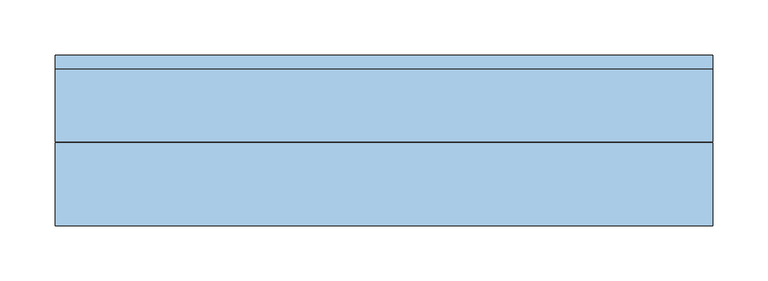
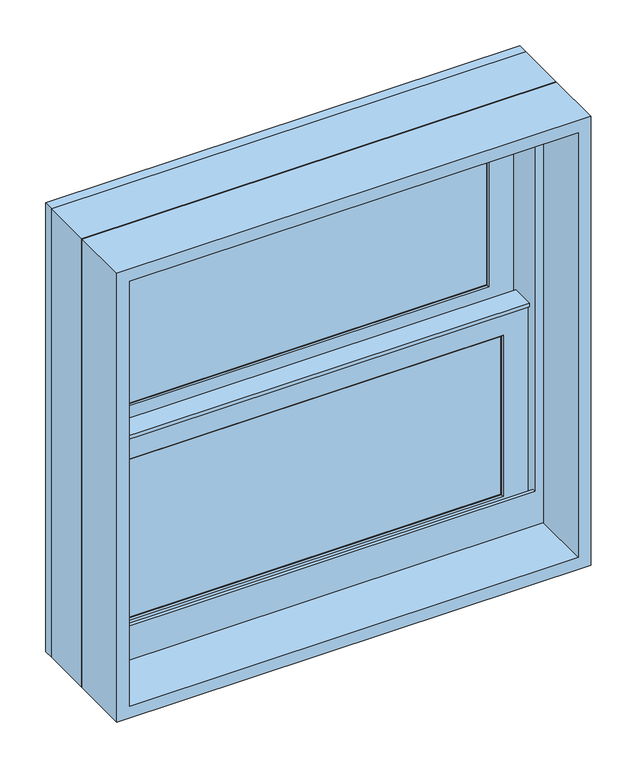
"""IFC4 building model written with IfcOpenShell, lengths in millimetres: window geometry, Window-Double_Hung-Marvin-Essential : ESDH2020."""

import ifcopenshell
import ifcopenshell.guid

model = None  # the IFC model being written
_history = None  # IfcOwnerHistory: only IFC2X3 demands one
_inside = {}  # id of a spatial element -> (the spatial element, [elements in it])
_under = {}  # id of a project, library or spatial element -> (it, [spatial elements below it])
_declared = {}  # id of a project -> (the project, [libraries it declares])
_typed = {}  # id of a type object -> (the type object, [elements of that type])
_made_of = {}  # id of a material, layer set ... -> (it, [elements and type objects made of it])


def new_model(schema):
    """Start an empty IFC model of exactly this schema.

    Asked for "IFC4X3", IfcOpenShell would pick the latest addendum, in which some entities
    have other attributes; the version numbers below select the first issue.
    IFC2X3 requires an IfcOwnerHistory on every rooted entity: one is made here for all.
    """
    global model, _history
    if schema == "IFC4X3":
        model = ifcopenshell.file(schema_version=(4, 3, 0, 0))
    else:
        model = ifcopenshell.file(schema=schema)
    _inside.clear()
    _under.clear()
    _declared.clear()
    _typed.clear()
    _made_of.clear()
    _history = None
    if model.schema == "IFC2X3":
        org = make("IfcOrganization", Name="unknown")
        user = make(
            "IfcPersonAndOrganization",
            ThePerson=make("IfcPerson", FamilyName="unknown"),
            TheOrganization=org,
        )
        app = make(
            "IfcApplication",
            ApplicationDeveloper=org,
            Version="unknown",
            ApplicationFullName="unknown",
            ApplicationIdentifier="unknown",
        )
        _history = make(
            "IfcOwnerHistory",
            OwningUser=user,
            OwningApplication=app,
            ChangeAction="ADDED",
            CreationDate=0,
        )
    return model


def make(cls, **values):
    """One entity of the class cls with the attributes given. An attribute that is None is left unset."""
    return model.create_entity(
        cls, **{name: value for name, value in values.items() if value is not None}
    )


def rooted(cls, **values):
    """An entity with a GlobalId (a new one), such as an element, a storey or a relation."""
    return make(cls, GlobalId=ifcopenshell.guid.new(), OwnerHistory=_history, **values)


def si_unit(unit_type, name, prefix=None):
    """IfcSIUnit, for example si_unit("LENGTHUNIT", "METRE", prefix="MILLI")."""
    return make("IfcSIUnit", UnitType=unit_type, Prefix=prefix, Name=name)


def assignment(units):
    """IfcUnitAssignment: the units of a project."""
    return None if units is None else make("IfcUnitAssignment", Units=units)


def point(xyz):
    """IfcCartesianPoint."""
    return None if xyz is None else make("IfcCartesianPoint", Coordinates=xyz)


def direction(xyz):
    """IfcDirection."""
    return None if xyz is None else make("IfcDirection", DirectionRatios=xyz)


def frame(location, z_axis=None, x_axis=None):
    """IfcAxis2Placement3D, a coordinate frame: its origin and axes. An axis left out is left unset."""
    return make(
        "IfcAxis2Placement3D",
        Location=point(location),
        Axis=direction(z_axis),
        RefDirection=direction(x_axis),
    )


def origin():
    """The frame at (0, 0, 0) with its axes left unset."""
    return frame((0.0, 0.0, 0.0))


def place(relative_to, where):
    """IfcLocalPlacement: puts the frame where relative to a parent placement (None: the world)."""
    return make(
        "IfcLocalPlacement", PlacementRelTo=relative_to, RelativePlacement=where
    )


def context(
    kind, dimensions, precision=None, world=None, true_north=None, identifier=None
):
    """IfcGeometricRepresentationContext, for example the 3D "Model" context."""
    return make(
        "IfcGeometricRepresentationContext",
        ContextIdentifier=identifier,
        ContextType=kind,
        CoordinateSpaceDimension=dimensions,
        Precision=precision,
        WorldCoordinateSystem=world,
        TrueNorth=true_north,
    )


def project(units=None, contexts=None):
    """IfcProject with its units and contexts."""
    return rooted(
        "IfcProject",
        Name="project",
        RepresentationContexts=contexts,
        UnitsInContext=assignment(units),
    )


def spatial(cls, under=None, at=None, **own):
    """A site, building, storey or space (cls), placed at a placement, below another one or the project."""
    s = rooted(cls, ObjectPlacement=at, **own)
    if under is not None:
        _under.setdefault(under.id(), (under, []))[1].append(s)
    return s


def polyline(points):
    """IfcPolyline through the points."""
    return make("IfcPolyline", Points=[point(p) for p in points])


def outline(outer, holes=None, kind="AREA"):
    """IfcArbitraryClosedProfileDef: a profile drawn as a closed curve; with holes, ...WithVoids."""
    if holes is None:
        return make("IfcArbitraryClosedProfileDef", ProfileType=kind, OuterCurve=outer)
    return make(
        "IfcArbitraryProfileDefWithVoids",
        ProfileType=kind,
        OuterCurve=outer,
        InnerCurves=holes,
    )


def extrude(swept, where, along, depth):
    """IfcExtrudedAreaSolid: the profile swept, set in the frame where, extruded along a direction by depth."""
    return make(
        "IfcExtrudedAreaSolid",
        SweptArea=swept,
        Position=where,
        ExtrudedDirection=direction(along),
        Depth=depth,
    )


def faces_of(points, faces, orient=None, outer=None):
    """IfcFace entities. A face is a list of loops; a loop is a list of indices into points, from 0.

    orient and outer hold one flag for each loop. By default every Orientation is true, the
    first loop of a face is its IfcFaceOuterBound and the others are IfcFaceBound.
    """
    made = []
    for i, loops in enumerate(faces):
        bounds = []
        for j, loop in enumerate(loops):
            is_outer = j == 0 if outer is None else outer[i][j]
            bounds.append(
                make(
                    "IfcFaceOuterBound" if is_outer else "IfcFaceBound",
                    Bound=make("IfcPolyLoop", Polygon=[points[k] for k in loop]),
                    Orientation=True if orient is None else orient[i][j],
                )
            )
        made.append(make("IfcFace", Bounds=bounds))
    return made


def faceted_brep(points, faces, orient=None, outer=None, voids=None):
    """IfcFacetedBrep: a solid bounded by flat faces; with voids (closed shells), ...WithVoids."""
    shared = [point(p) for p in points]
    hull = make("IfcClosedShell", CfsFaces=faces_of(shared, faces, orient, outer))
    if voids is None:
        return make("IfcFacetedBrep", Outer=hull)
    return make(
        "IfcFacetedBrepWithVoids",
        Outer=hull,
        Voids=[
            make(cls, CfsFaces=faces_of(shared, fs, o, b)) for cls, fs, o, b in voids
        ],
    )


def shape(context_of_items, identifier, shape_type, items):
    """IfcShapeRepresentation: the items that make up one representation, for example the "Body"."""
    return make(
        "IfcShapeRepresentation",
        ContextOfItems=context_of_items,
        RepresentationIdentifier=identifier,
        RepresentationType=shape_type,
        Items=items,
    )


def source(mapping_origin, context_of_items, identifier, shape_type, items):
    """IfcRepresentationMap: a shape defined once, which mapped items show again and again."""
    return make(
        "IfcRepresentationMap",
        MappingOrigin=mapping_origin,
        MappedRepresentation=shape(context_of_items, identifier, shape_type, items),
    )


def transform(
    local_origin,
    x_axis=None,
    y_axis=None,
    z_axis=None,
    scale=None,
    scale2=None,
    scale3=None,
    uniform=True,
):
    """IfcCartesianTransformationOperator3D, or its non-uniform kind. x_axis, y_axis, z_axis: its Axis1, 2, 3."""
    if uniform:
        return make(
            "IfcCartesianTransformationOperator3D",
            Axis1=direction(x_axis),
            Axis2=direction(y_axis),
            LocalOrigin=point(local_origin),
            Scale=scale,
            Axis3=direction(z_axis),
        )
    return make(
        "IfcCartesianTransformationOperator3DnonUniform",
        Axis1=direction(x_axis),
        Axis2=direction(y_axis),
        LocalOrigin=point(local_origin),
        Scale=scale,
        Axis3=direction(z_axis),
        Scale2=scale2,
        Scale3=scale3,
    )


def mapped(mapping_source, mapping_target):
    """IfcMappedItem: shows the shape of a source again, moved by a transform."""
    return make(
        "IfcMappedItem", MappingSource=mapping_source, MappingTarget=mapping_target
    )


def made_of(thing, what):
    """Note that an element or type object is made of a material, layer set ...; save() writes the relation."""
    if what is not None:
        _made_of.setdefault(what.id(), (what, []))[1].append(thing)
    return thing


def element(
    cls,
    number,
    at=None,
    inside=None,
    cuts=None,
    type_object=None,
    material=None,
    context=None,
    identifier="Body",
    shape_type=None,
    held_by="IfcProductDefinitionShape",
    body=None,
    shapes=None,
    **own,
):
    """One element of the class cls, such as IfcWall. Its Tag is "e" and its number.

    at: its placement. inside: the storey or other place that contains it. cuts: it is an
    opening in that element (IfcRelVoidsElement). A single representation is given by context,
    identifier, shape_type and body (its items); several are given by shapes. held_by: the class
    of the entity that holds the representations. save() writes the other relations.
    """
    e = rooted(cls, Tag="e%d" % number, ObjectPlacement=at, **own)
    if body is not None:
        shapes = [shape(context, identifier, shape_type, body)]
    if shapes is not None:
        e.Representation = make(held_by, Representations=shapes)
    if inside is not None:
        _inside.setdefault(inside.id(), (inside, []))[1].append(e)
    if cuts is not None:
        rooted(
            "IfcRelVoidsElement", RelatingBuildingElement=cuts, RelatedOpeningElement=e
        )
    if type_object is not None:
        _typed.setdefault(type_object.id(), (type_object, []))[1].append(e)
    return made_of(e, material)


def aggregate(whole, parts):
    """IfcRelAggregates: a whole, such as a stair, and the parts it consists of."""
    return rooted("IfcRelAggregates", RelatingObject=whole, RelatedObjects=parts)


def save(model, path):
    """Write the relations noted so far, then the file.

    IfcRelAggregates (storeys below a building ...), IfcRelContainedInSpatialStructure (elements
    in a storey), IfcRelDefinesByType, IfcRelAssociatesMaterial and IfcRelDeclares: one each for
    every whole, place, type object, material and project.
    """
    for whole, parts in _under.values():
        aggregate(whole, parts)
    for where, things in _inside.values():
        rooted(
            "IfcRelContainedInSpatialStructure",
            RelatedElements=things,
            RelatingStructure=where,
        )
    for kind, things in _typed.values():
        rooted("IfcRelDefinesByType", RelatedObjects=things, RelatingType=kind)
    for what, things in _made_of.values():
        rooted("IfcRelAssociatesMaterial", RelatedObjects=things, RelatingMaterial=what)
    for by, libraries in _declared.values():
        rooted("IfcRelDeclares", RelatingContext=by, RelatedDefinitions=libraries)
    model.write(path)


def window_35121546(model_context):
    return source(origin(), model_context, "Body", "SolidModel", [
        extrude(outline(polyline([(89.9583333, 20.6375), (89.9583333, 15.875), (70.9083333, 15.875), (70.9083333, 20.6375), (89.9583333, 20.6375)])), frame((0.0, 0.0, 1898.65), z_axis=(0.0, 0.0, 1.0), x_axis=(1.0, 0.0, 0.0)), (0.0, 0.0, 1.0), 222.25),
        extrude(outline(polyline([(-70.9083333, 20.6375), (-70.9083333, 15.875), (-89.9583333, 15.875), (-89.9583333, 20.6375), (-70.9083333, 20.6375)])), frame((0.0, 0.0, 1898.65), z_axis=(0.0, 0.0, 1.0), x_axis=(1.0, 0.0, 0.0)), (0.0, 0.0, 1.0), 222.25),
        extrude(outline(polyline([(241.3, 20.6375), (241.3, 15.875), (-241.3, 15.875), (-241.3, 20.6375), (241.3, 20.6375)])), frame((0.0, 0.0, 2000.25), z_axis=(0.0, 0.0, 1.0), x_axis=(1.0, 0.0, 0.0)), (0.0, 0.0, 1.0), 19.05),
        extrude(outline(polyline([(-89.9583333, 46.83125), (-89.9583333, 51.59375), (-70.9083333, 51.59375), (-70.9083333, 46.83125), (-89.9583333, 46.83125)])), frame((0.0, 0.0, 2159.0), z_axis=(0.0, 0.0, 1.0), x_axis=(1.0, 0.0, 0.0)), (0.0, 0.0, 1.0), 222.25),
        extrude(outline(polyline([(70.9083333, 46.83125), (70.9083333, 51.59375), (89.9583333, 51.59375), (89.9583333, 46.83125), (70.9083333, 46.83125)])), frame((0.0, 0.0, 2159.0), z_axis=(0.0, 0.0, 1.0), x_axis=(1.0, 0.0, 0.0)), (0.0, 0.0, 1.0), 222.25),
        extrude(outline(polyline([(-241.3, 46.83125), (-241.3, 51.59375), (241.3, 51.59375), (241.3, 46.83125), (-241.3, 46.83125)])), frame((0.0, 0.0, 2260.6), z_axis=(0.0, 0.0, 1.0), x_axis=(1.0, 0.0, 0.0)), (0.0, 0.0, 1.0), 19.05),
        extrude(outline(polyline([(89.9583333, 20.6375), (70.9083333, 20.6375), (70.9083333, 25.4), (89.9583333, 25.4), (89.9583333, 20.6375)])), frame((0.0, 0.0, 1898.65), z_axis=(0.0, 0.0, 1.0), x_axis=(1.0, 0.0, 0.0)), (0.0, 0.0, 1.0), 222.25),
        extrude(outline(polyline([(-70.9083333, 20.6375), (-89.9583333, 20.6375), (-89.9583333, 25.4), (-70.9083333, 25.4), (-70.9083333, 20.6375)])), frame((0.0, 0.0, 1898.65), z_axis=(0.0, 0.0, 1.0), x_axis=(1.0, 0.0, 0.0)), (0.0, 0.0, 1.0), 222.25),
        extrude(outline(polyline([(241.3, 20.6375), (-241.3, 20.6375), (-241.3, 25.4), (241.3, 25.4), (241.3, 20.6375)])), frame((0.0, 0.0, 2000.25), z_axis=(0.0, 0.0, 1.0), x_axis=(1.0, 0.0, 0.0)), (0.0, 0.0, 1.0), 19.05),
        extrude(outline(polyline([(-89.9583333, 56.35625), (-70.9083333, 56.35625), (-70.9083333, 51.59375), (-89.9583333, 51.59375), (-89.9583333, 56.35625)])), frame((0.0, 0.0, 2159.0), z_axis=(0.0, 0.0, 1.0), x_axis=(1.0, 0.0, 0.0)), (0.0, 0.0, 1.0), 222.25),
        extrude(outline(polyline([(70.9083333, 56.35625), (89.9583333, 56.35625), (89.9583333, 51.59375), (70.9083333, 51.59375), (70.9083333, 56.35625)])), frame((0.0, 0.0, 2159.0), z_axis=(0.0, 0.0, 1.0), x_axis=(1.0, 0.0, 0.0)), (0.0, 0.0, 1.0), 222.25),
        extrude(outline(polyline([(-241.3, 56.35625), (241.3, 56.35625), (241.3, 51.59375), (-241.3, 51.59375), (-241.3, 56.35625)])), frame((0.0, 0.0, 2260.6), z_axis=(0.0, 0.0, 1.0), x_axis=(1.0, 0.0, 0.0)), (0.0, 0.0, 1.0), 19.05),
        faceted_brep([(-268.2875, 5.6780605, 2150.9351748), (-268.2875, 5.6780605, 2146.3), (268.2875, 5.6780605, 2146.3), (268.2875, 5.6780605, 2150.9351748), (-268.2875, 34.8118605, 2150.9351748), (268.2875, 34.8118605, 2150.9351748), (268.2875, 34.8118605, 2146.3), (-268.2875, 34.8118605, 2146.3), (-268.2875, 30.1625, 2146.3), (-268.2875, 30.1625, 1871.6625), (-268.2875, 8.9241104, 1871.6625), (-268.2875, 8.9241104, 2146.3), (268.2875, 8.9241104, 2146.3), (268.2875, 30.1625, 2146.3), (268.2875, 8.9241104, 1871.6625), (268.2875, 30.1625, 1871.6625), (-252.4034752, 11.90625, 2132.0034752), (-252.4034752, 30.1625, 2132.0034752), (252.4034752, 30.1625, 2132.0034752), (252.4034752, 11.90625, 2132.0034752), (-235.74375, 10.4662439, 2115.34375), (-235.74375, 11.90625, 2115.34375), (235.74375, 11.90625, 2115.34375), (235.74375, 10.4662439, 2115.34375), (237.2858834, 8.9241104, 2116.8858834), (-237.2858834, 8.9241104, 2116.8858834), (252.4034752, 30.1625, 1887.5465248), (252.4034752, 11.90625, 1887.5465248), (235.74375, 11.90625, 1904.20625), (235.74375, 10.4662439, 1904.20625), (237.2858834, 8.9241104, 1902.6641166), (-252.4034752, 30.1625, 1887.5465248), (-252.4034752, 11.90625, 1887.5465248), (-235.74375, 11.90625, 1904.20625), (-235.74375, 10.4662439, 1904.20625), (-237.2858834, 8.9241104, 1902.6641166)], [[[0, 1, 2, 3]], [[4, 5, 6, 7]], [[1, 0, 4, 7, 8, 9, 10, 11]], [[2, 1, 11, 12]], [[7, 6, 13, 8]], [[3, 2, 12, 14, 15, 13, 6, 5]], [[0, 3, 5, 4]], [[16, 17, 18, 19]], [[20, 21, 22, 23]], [[20, 23, 24, 25]], [[19, 18, 26, 27]], [[23, 22, 28, 29]], [[24, 23, 29, 30]], [[27, 26, 31, 32]], [[29, 28, 33, 34]], [[30, 29, 34, 35]], [[15, 14, 10, 9]], [[15, 9, 8, 13], [18, 17, 31, 26]], [[17, 16, 32, 31]], [[16, 19, 27, 32], [22, 21, 33, 28]], [[21, 20, 34, 33]], [[20, 25, 35, 34]], [[10, 14, 12, 11], [25, 24, 30, 35]]]),
        extrude(outline(polyline([(38.5955581, 2132.0125), (33.5778968, 2132.0125), (33.5778968, 2133.6), (39.9405976, 2133.6), (39.9405976, 2132.0125), (61.515625, 2132.0125), (47.6307501, 2128.6975159), (38.5955581, 2128.6975159), (38.5955581, 2132.0125)])), frame((-268.2875, 0.0, 0.0), z_axis=(1.0, 0.0, 0.0), x_axis=(0.0, 1.0, 0.0)), (0.0, 0.0, 1.0), 536.575),
        faceted_brep([(298.45, 0.0, 1841.5), (298.45, 0.0, 2438.4), (-298.45, 0.0, 2438.4), (-298.45, 0.0, 1841.5), (272.25625, 0.0, 1902.61875), (-272.25625, 0.0, 1902.61875), (-272.25625, 0.0, 2412.20625), (272.25625, 0.0, 2412.20625), (272.25625, 3.96875, 1841.5), (-272.25625, 3.96875, 1841.5), (-272.25625, 3.96875, 1902.61875), (272.25625, 3.96875, 1902.61875), (-298.45, 65.6828125, 1841.5), (-272.25625, 65.6828125, 1841.5), (272.25625, 65.6828125, 1841.5), (298.45, 65.6828125, 1841.5), (-298.45, 65.6828125, 2438.4), (298.45, 65.6828125, 2438.4), (272.25625, 65.6828125, 2412.20625), (-272.25625, 65.6828125, 2412.20625)], [[[0, 1, 2, 3], [4, 5, 6, 7]], [[8, 9, 10, 11]], [[5, 4, 11, 10]], [[0, 3, 12, 13, 9, 8, 14, 15]], [[13, 12, 16, 17, 15, 14, 18, 19]], [[13, 19, 6, 5, 10, 9]], [[7, 6, 19, 18]], [[18, 14, 8, 11, 4, 7]], [[1, 0, 15, 17]], [[2, 1, 17, 16]], [[3, 2, 16, 12]]]),
        faceted_brep([(272.25625, 30.1625, 2139.95), (270.66875, 30.1625, 2139.95), (270.66875, 30.1625, 1865.8544613), (272.25625, 30.1625, 1865.8544613), (-270.66875, 30.1625, 2139.95), (-272.25625, 30.1625, 2139.95), (-272.25625, 30.1625, 1865.8544613), (-270.66875, 30.1625, 1865.8544613), (270.66875, 63.5, 2139.95), (272.25625, 63.5, 2139.95), (272.25625, 63.5, 1859.3743077), (270.66875, 63.5, 1859.3743077), (-272.25625, 63.5, 2139.95), (-270.66875, 63.5, 2139.95), (-270.66875, 63.5, 1859.3743077), (-272.25625, 63.5, 1859.3743077), (283.5108932, 3.96875, 1870.9460105), (283.5108932, 3.96875, 1841.5), (283.5108932, 65.6828125, 1841.5), (283.5108932, 65.6828125, 1858.950012), (-283.5108932, 3.96875, 1841.5), (-283.5108932, 3.96875, 1870.9460105), (-283.5108932, 65.6828125, 1858.950012), (-283.5108932, 65.6828125, 1841.5), (283.5108932, 78.58125, 1856.4428097), (-283.5108932, 78.58125, 1856.4428097), (-281.4971252, 68.2348864, 1858.4539391), (-263.53135, 68.2348864, 1858.4539391), (-263.53135, 65.6828125, 1858.950012), (263.53135, 65.6828125, 1858.950012), (263.53135, 68.2348864, 1858.4539391), (281.4971252, 68.2348864, 1858.4539391), (-298.45, 65.6828125, 1841.5), (-298.45, 78.5948249, 1841.5), (298.45, 78.5948249, 1841.5), (298.45, 65.6828125, 1841.5), (-298.45, 78.58125, 2438.4), (298.45, 78.58125, 2438.4), (283.5108932, 78.58125, 2423.4608932), (-283.5108932, 78.58125, 2423.4608932), (-298.45, 65.6828125, 2438.4), (-281.4971252, 68.2348864, 2421.4471252), (281.4971252, 68.2348864, 2421.4471252), (263.53135, 68.2348864, 2403.48135), (-263.53135, 68.2348864, 2403.48135), (-263.53135, 65.6828125, 2403.48135), (263.53135, 65.6828125, 2403.48135), (298.45, 65.6828125, 2438.4)], [[[0, 1, 2, 3]], [[4, 5, 6, 7]], [[8, 9, 10, 11]], [[12, 13, 14, 15]], [[1, 8, 11, 2]], [[9, 0, 3, 10]], [[1, 0, 9, 8]], [[5, 4, 13, 12]], [[5, 12, 15, 6]], [[13, 4, 7, 14]], [[16, 17, 18, 19]], [[20, 21, 22, 23]], [[24, 25, 26, 27, 28, 22, 21, 16, 19, 29, 30, 31], [3, 2, 11, 10], [7, 6, 15, 14]], [[17, 16, 21, 20]], [[17, 20, 23, 32, 33, 34, 35, 18]], [[34, 33, 36, 37], [25, 24, 38, 39]], [[33, 32, 40, 36]], [[39, 41, 26, 25]], [[41, 42, 31, 30, 43, 44, 27, 26]], [[44, 45, 28, 27]], [[40, 32, 23, 22, 28, 45, 46, 29, 19, 18, 35, 47]], [[36, 40, 47, 37]], [[39, 38, 42, 41]], [[44, 43, 46, 45]], [[34, 37, 47, 35]], [[42, 38, 24, 31]], [[46, 43, 30, 29]]]),
        extrude(outline(polyline([(248.44375, 11.90625), (-248.44375, 11.90625), (-248.44375, 15.08125), (248.44375, 15.08125), (248.44375, 11.90625)])), frame((0.0, 0.0, 1891.50625), z_axis=(0.0, 0.0, 1.0), x_axis=(1.0, 0.0, 0.0)), (0.0, 0.0, 1.0), 236.5375),
        extrude(outline(polyline([(248.44375, 42.8625), (-248.44375, 42.8625), (-248.44375, 46.0375), (248.44375, 46.0375), (248.44375, 42.8625)])), frame((0.0, 0.0, 2151.85625), z_axis=(0.0, 0.0, 1.0), x_axis=(1.0, 0.0, 0.0)), (0.0, 0.0, 1.0), 236.5375),
        faceted_brep([(-235.74375, 31.194477, 2115.34375), (-237.2858834, 32.7366104, 2116.8858834), (237.2858834, 32.7366104, 2116.8858834), (235.74375, 31.194477, 2115.34375), (-235.74375, 30.1625, 2115.34375), (235.74375, 30.1625, 2115.34375), (-268.2875, 32.7366104, 2147.8875), (-268.2875, 30.1625, 2147.8875), (268.2875, 30.1625, 2147.8875), (268.2875, 32.7366104, 2147.8875), (237.2858834, 32.7366104, 1902.6641166), (235.74375, 31.194477, 1904.20625), (235.74375, 30.1625, 1904.20625), (268.2875, 30.1625, 1871.6625), (268.2875, 32.7366104, 1871.6625), (-237.2858834, 32.7366104, 1902.6641166), (-235.74375, 31.194477, 1904.20625), (-235.74375, 30.1625, 1904.20625), (-268.2875, 30.1625, 1871.6625), (-268.2875, 32.7366104, 1871.6625)], [[[0, 1, 2, 3]], [[4, 0, 3, 5]], [[6, 7, 8, 9]], [[3, 2, 10, 11]], [[5, 3, 11, 12]], [[9, 8, 13, 14]], [[11, 10, 15, 16]], [[12, 11, 16, 17]], [[14, 13, 18, 19]], [[9, 14, 19, 6], [1, 15, 10, 2]], [[16, 15, 1, 0]], [[17, 16, 0, 4]], [[7, 18, 13, 8], [5, 12, 17, 4]], [[19, 18, 7, 6]]]),
        faceted_brep([(-252.4034752, 42.8625, 2392.3534752), (-252.4034752, 61.11875, 2392.3534752), (252.4034752, 61.11875, 2392.3534752), (252.4034752, 42.8625, 2392.3534752), (-235.74375, 41.4224939, 2375.69375), (-235.74375, 42.8625, 2375.69375), (235.74375, 42.8625, 2375.69375), (235.74375, 41.4224939, 2375.69375), (-237.2858834, 39.8803604, 2377.2358834), (237.2858834, 39.8803604, 2377.2358834), (-268.2875, 61.11875, 2408.2375), (-268.2875, 39.8803604, 2408.2375), (268.2875, 39.8803604, 2408.2375), (268.2875, 61.11875, 2408.2375), (252.4034752, 61.11875, 2147.8965248), (252.4034752, 42.8625, 2147.8965248), (235.74375, 42.8625, 2164.55625), (235.74375, 41.4224939, 2164.55625), (237.2858834, 39.8803604, 2163.0141166), (268.2875, 39.8803604, 2132.0125), (268.2875, 61.11875, 2132.0125), (-252.4034752, 61.11875, 2147.8965248), (-252.4034752, 42.8625, 2147.8965248), (-235.74375, 42.8625, 2164.55625), (-235.74375, 41.4224939, 2164.55625), (-237.2858834, 39.8803604, 2163.0141166), (-268.2875, 39.8803604, 2132.0125), (-268.2875, 61.11875, 2132.0125)], [[[0, 1, 2, 3]], [[4, 5, 6, 7]], [[8, 4, 7, 9]], [[10, 11, 12, 13]], [[3, 2, 14, 15]], [[7, 6, 16, 17]], [[9, 7, 17, 18]], [[13, 12, 19, 20]], [[15, 14, 21, 22]], [[17, 16, 23, 24]], [[18, 17, 24, 25]], [[20, 19, 26, 27]], [[13, 20, 27, 10], [1, 21, 14, 2]], [[22, 21, 1, 0]], [[3, 15, 22, 0], [5, 23, 16, 6]], [[24, 23, 5, 4]], [[25, 24, 4, 8]], [[11, 26, 19, 12], [9, 18, 25, 8]], [[27, 26, 11, 10]]]),
        faceted_brep([(-268.2875, 61.11875, 2132.0125), (-268.2875, 63.6928604, 2132.0125), (268.2875, 63.6928604, 2132.0125), (268.2875, 61.11875, 2132.0125), (-235.74375, 62.150727, 2164.55625), (-235.74375, 61.11875, 2164.55625), (235.74375, 61.11875, 2164.55625), (235.74375, 62.150727, 2164.55625), (-237.2858834, 63.6928604, 2163.0141166), (237.2858834, 63.6928604, 2163.0141166), (268.2875, 63.6928604, 2408.2375), (268.2875, 61.11875, 2408.2375), (235.74375, 61.11875, 2375.69375), (235.74375, 62.150727, 2375.69375), (237.2858834, 63.6928604, 2377.2358834), (-268.2875, 63.6928604, 2408.2375), (-268.2875, 61.11875, 2408.2375), (-235.74375, 61.11875, 2375.69375), (-235.74375, 62.150727, 2375.69375), (-237.2858834, 63.6928604, 2377.2358834)], [[[0, 1, 2, 3]], [[4, 5, 6, 7]], [[8, 4, 7, 9]], [[3, 2, 10, 11]], [[7, 6, 12, 13]], [[9, 7, 13, 14]], [[11, 10, 15, 16]], [[13, 12, 17, 18]], [[14, 13, 18, 19]], [[16, 15, 1, 0]], [[3, 11, 16, 0], [5, 17, 12, 6]], [[18, 17, 5, 4]], [[19, 18, 4, 8]], [[1, 15, 10, 2], [9, 14, 19, 8]]]),
        extrude(outline(polyline([(248.44375, 26.19375), (-248.44375, 26.19375), (-248.44375, 30.1625), (248.44375, 30.1625), (248.44375, 26.19375)])), frame((0.0, 0.0, 1891.50625), z_axis=(0.0, 0.0, 1.0), x_axis=(1.0, 0.0, 0.0)), (0.0, 0.0, 1.0), 236.5375),
        extrude(outline(polyline([(248.44375, 57.15), (-248.44375, 57.15), (-248.44375, 61.11875), (248.44375, 61.11875), (248.44375, 57.15)])), frame((0.0, 0.0, 2151.85625), z_axis=(0.0, 0.0, 1.0), x_axis=(1.0, 0.0, 0.0)), (0.0, 0.0, 1.0), 236.5375),
        extrude(outline(polyline([(2438.4, 298.45), (2438.4, -298.45), (1841.5, -298.45), (1841.5, 298.45), (2438.4, 298.45)]), holes=[polyline([(2422.525, 282.575), (1857.375, 282.575), (1857.375, -282.575), (2422.525, -282.575), (2422.525, 282.575)])]), frame((0.0, -76.2, 0.0), z_axis=(0.0, 1.0, 0.0), x_axis=(0.0, 0.0, 1.0)), (0.0, 0.0, 1.0), 75.40625),
    ])


if __name__ == "__main__":
    model = new_model("IFC4")
    model_context = context("Model", 3, world=origin())
    ifc_project = project(units=[si_unit("LENGTHUNIT", "METRE", prefix="MILLI")], contexts=[model_context])
    site = spatial("IfcSite", under=ifc_project)
    building = spatial("IfcBuilding", under=site)
    placement = place(None, origin())
    window_shape = window_35121546(model_context)
    element("IfcWindow", 1, ObjectType="Window-Double_Hung-Marvin-Essential : ESDH2020", at=placement, inside=building, context=model_context, shape_type="MappedRepresentation", body=[
        mapped(window_shape, transform((0.0, 0.0, 0.0), x_axis=(1.0, 0.0, 0.0), y_axis=(0.0, 1.0, 0.0), z_axis=(0.0, 0.0, 1.0))),
    ])
    save(model, "model.ifc")

# Revit data of these elements
# Type "Window-Double_Hung-Marvin-Essential : ESDH2020"
#   Type Mark = "20"
#   Window Type = "Essential Double Hung"
#   Product data url = "https://bimobject.com/marvin-windows-and-doors/product/marvin-dhwau"
#   Product Guid = "c4a96547-874c-4385-91dc-a058adc19d98"
#   Frame = "All Ultrex"
#   Egress Window = "No"
#   URL = "www.marvin.com"
#   Model = "ESDH2020"
#   Manufacturer = "Marvin Windows and Doors"
#   Label Egress = ""
#   Glass Type = "IG Low E II with Argon"
#   Design Pressure = "DP50"
#   Description = "2424 DBHG"
#   Analytic Construction = "<None>"
#   Prairie Corner Width = 0' - 4"
#   Prairie Corner Height = 0' - 4"
#   Egress Width = 1' - 8 9/16"
#   Egress Height = 0' - 7 27/128"
#   Rough Width = 2' - 0"
#   Rough Height = 2' - 0"
#   Nominal Width = 2' - 0"
#   Nominal Height = 2' - 0"
#   Inset to Installation Flange [instance default] = 0' - 1"
#   Height = 1' - 11 1/2"
#   Egress Area = 1.02969 SF
#   Default Head Height = 8' - 0"
#   Width = 1' - 11 1/2"
#   Daylight Area = 2.14307 SF
#   DLO Width = 1' - 6 9/16"
#   DLO Height = 0' - 8 5/16"
#   Muntins Top Sash = yes
#   Lites Wide Top Sash = 3
#   Lites Wide Bottom Sash = 3
#   Lites High Top Sash = 2
#   Lites High Bottom Sash = 2
#   Lite Cut Prairie 9 = no
#   Lite Cut HV Grid = yes
#   Muntins Bottom Sash = yes
#   Label Visibility = no
#   Jamb Extension Visibility = yes
#   Edition number = 1
#   Interior Material = Ultrex-Marvin-Stonewhite
#   Glazing Material = Glass-Marvin-IG Low E II with Argon
#   Cladding Material = Ultrex-Marvin-Pebblegray
#   Wall Closure = (empty or 0)
#   Assembly Code = ""
# Element 1 (IfcWindow, "Window-Double_Hung-Marvin-Essential : ESDH2020")
#   Materials on its faces: "Ultrex-Marvin-Pebblegray", "Ultrex-Marvin-Stonewhite", "Glass-Marvin-IG Low E II with Argon"
# Materials
#   "Ultrex-Marvin-Stonewhite": class "Paint", colour RGB 250 251 245, transparency 0
#   "Glass-Marvin-IG Low E II with Argon": class "Glass", colour RGB 0 128 192, transparency 0.85
#   "Ultrex-Marvin-Pebblegray": class "Paint", colour RGB 189 185 173, transparency 0
